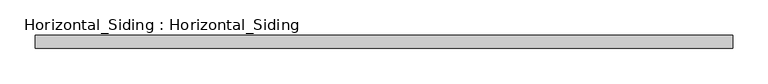
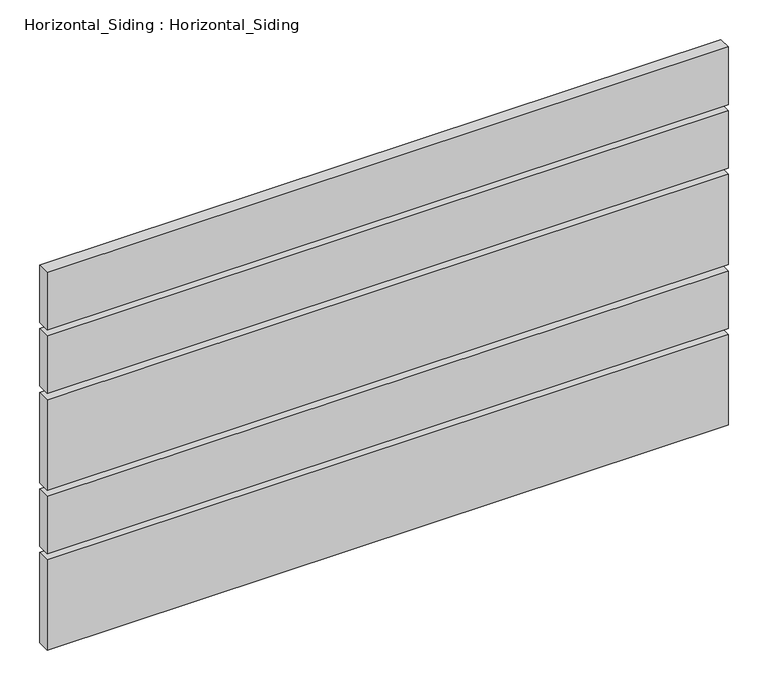
"""IFC4 building model written with IfcOpenShell, lengths in millimetres: plate geometry, Horizontal_Siding : Horizontal_Siding."""

from ifc_helpers import new_model, si_unit, frame, origin, place, context, project, spatial, polyline, outline, extrude, source, transform, mapped, element, save


def horizontal_siding_horizontal_siding_aa6357ad(model_context):
    return source(origin(), model_context, "Body", "SweptSolid", [
        extrude(outline(polyline([(497.8365389, -19.05), (-497.8365389, -19.05), (-497.8365389, 0.0), (497.8365389, 0.0), (497.8365389, -19.05)])), frame((0.0, 0.0, 9.525), z_axis=(0.0, 0.0, 1.0), x_axis=(1.0, 0.0, 0.0)), (0.0, 0.0, 1.0), 139.7),
        extrude(outline(polyline([(497.8365389, -19.05), (-497.8365389, -19.05), (-497.8365389, 0.0), (497.8365389, 0.0), (497.8365389, -19.05)])), frame((0.0, 0.0, 158.75), z_axis=(0.0, 0.0, 1.0), x_axis=(1.0, 0.0, 0.0)), (0.0, 0.0, 1.0), 88.9),
        extrude(outline(polyline([(497.8365389, -19.05), (-497.8365389, -19.05), (-497.8365389, 0.0), (497.8365389, 0.0), (497.8365389, -19.05)])), frame((0.0, 0.0, 257.175), z_axis=(0.0, 0.0, 1.0), x_axis=(1.0, 0.0, 0.0)), (0.0, 0.0, 1.0), 139.7),
        extrude(outline(polyline([(497.8365389, -19.05), (-497.8365389, -19.05), (-497.8365389, 0.0), (497.8365389, 0.0), (497.8365389, -19.05)])), frame((0.0, 0.0, 406.4), z_axis=(0.0, 0.0, 1.0), x_axis=(1.0, 0.0, 0.0)), (0.0, 0.0, 1.0), 88.9),
        extrude(outline(polyline([(497.8365389, -19.05), (-497.8365389, -19.05), (-497.8365389, 0.0), (497.8365389, 0.0), (497.8365389, -19.05)])), frame((0.0, 0.0, 504.825), z_axis=(0.0, 0.0, 1.0), x_axis=(1.0, 0.0, 0.0)), (0.0, 0.0, 1.0), 88.9),
    ])


if __name__ == "__main__":
    model = new_model("IFC4")
    model_context = context("Model", 3, world=origin())
    ifc_project = project(units=[si_unit("LENGTHUNIT", "METRE", prefix="MILLI")], contexts=[model_context])
    site = spatial("IfcSite", under=ifc_project)
    building = spatial("IfcBuilding", under=site)
    placement = place(None, origin())
    horizontal_siding_horizontal_siding_shape = horizontal_siding_horizontal_siding_aa6357ad(model_context)
    element("IfcPlate", 1, ObjectType="Horizontal_Siding : Horizontal_Siding", at=placement, inside=building, context=model_context, shape_type="MappedRepresentation", body=[
        mapped(horizontal_siding_horizontal_siding_shape, transform((0.0, 0.0, 0.0), x_axis=(1.0, 0.0, 0.0), y_axis=(0.0, 1.0, 0.0), z_axis=(0.0, 0.0, 1.0))),
    ])
    save(model, "model.ifc")

# Revit data of these elements
# Type "Horizontal_Siding : Horizontal_Siding"
#   Analytic Construction = "<None>"
#   extend = 0' - 2 3/4"
#   Width_2 = 0' - 3 1/2"
#   Width_1 = 0' - 5 1/2"
#   Gap = 0' - 0 3/8"
#   Plank Material = SLOTTED WOOD FENCE (THERMALLY MODIFIED WOOD: ARBOR WOOD)\n(EXTERIOR STAIN : PENOFIN VERDE EXT. STAIN - COLOR: CEDAR)
# Element 1 (IfcPlate, "Horizontal_Siding : Horizontal_Siding")
#   Materials on its faces: "SLOTTED WOOD FENCE (THERMALLY MODIFIED WOOD: ARBOR WOOD)\n(EXTERIOR STAIN : PENOFIN VERDE EXT. STAIN - COLOR: CEDAR)"
# Materials
#   "SLOTTED WOOD FENCE (THERMALLY MODIFIED WOOD: ARBOR WOOD)\n(EXTERIOR STAIN : PENOFIN VERDE EXT. STAIN - COLOR: CEDAR)": class "Wood", colour RGB 164 134 123, transparency 0, Description = "Pinus Echinata", Cost = 0
